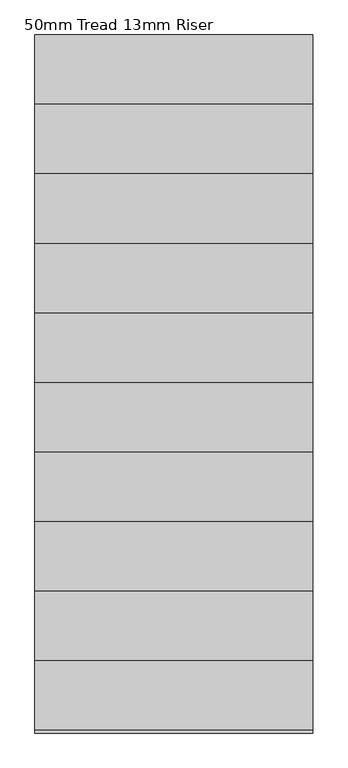
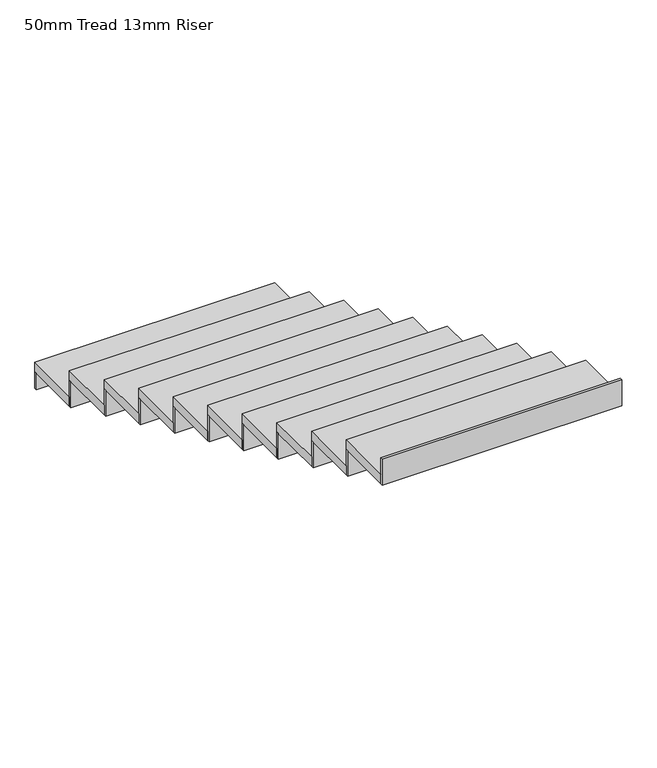
"""IFC4 building model written with IfcOpenShell, lengths in millimetres: stair flight geometry, 50mm Tread 13mm Riser."""

from ifc_helpers import new_model, si_unit, frame, origin, origin_with_axes, place, context, project, spatial, polyline, outline, extrude, source, transform, mapped, element, save


def stair_flight_50mm_tread_13mm_riser_f0aa37fc(model_context):
    return source(origin(), model_context, "Body", "SweptSolid", [
        extrude(outline(polyline([(21558.5156953, 793.6136739), (21558.5156953, 806.1136739), (22758.5156953, 806.1136739), (22758.5156953, 793.6136739), (21558.5156953, 793.6136739)])), origin_with_axes(), (0.0, 0.0, 1.0), 86.3636364),
        extrude(outline(polyline([(22758.5156953, 506.1136739), (21558.5156953, 506.1136739), (21558.5156953, 806.1136739), (22758.5156953, 806.1136739), (22758.5156953, 506.1136739)])), frame((0.0, 0.0, 86.3636364), z_axis=(0.0, 0.0, 1.0), x_axis=(1.0, 0.0, 0.0)), (0.0, 0.0, 1.0), 50.0),
        extrude(outline(polyline([(21558.5156953, 493.6136739), (21558.5156953, 506.1136739), (22758.5156953, 506.1136739), (22758.5156953, 493.6136739), (21558.5156953, 493.6136739)])), frame((0.0, 0.0, 86.3636364), z_axis=(0.0, 0.0, 1.0), x_axis=(1.0, 0.0, 0.0)), (0.0, 0.0, 1.0), 136.3636364),
        extrude(outline(polyline([(22758.5156953, 206.1136739), (21558.5156953, 206.1136739), (21558.5156953, 506.1136739), (22758.5156953, 506.1136739), (22758.5156953, 206.1136739)])), frame((0.0, 0.0, 222.7272727), z_axis=(0.0, 0.0, 1.0), x_axis=(1.0, 0.0, 0.0)), (0.0, 0.0, 1.0), 50.0),
        extrude(outline(polyline([(21558.5156953, 193.6136739), (21558.5156953, 206.1136739), (22758.5156953, 206.1136739), (22758.5156953, 193.6136739), (21558.5156953, 193.6136739)])), frame((0.0, 0.0, 222.7272727), z_axis=(0.0, 0.0, 1.0), x_axis=(1.0, 0.0, 0.0)), (0.0, 0.0, 1.0), 136.3636364),
        extrude(outline(polyline([(22758.5156953, -93.8863261), (21558.5156953, -93.8863261), (21558.5156953, 206.1136739), (22758.5156953, 206.1136739), (22758.5156953, -93.8863261)])), frame((0.0, 0.0, 359.0909091), z_axis=(0.0, 0.0, 1.0), x_axis=(1.0, 0.0, 0.0)), (0.0, 0.0, 1.0), 50.0),
        extrude(outline(polyline([(21558.5156953, -106.3863261), (21558.5156953, -93.8863261), (22758.5156953, -93.8863261), (22758.5156953, -106.3863261), (21558.5156953, -106.3863261)])), frame((0.0, 0.0, 359.0909091), z_axis=(0.0, 0.0, 1.0), x_axis=(1.0, 0.0, 0.0)), (0.0, 0.0, 1.0), 136.3636364),
        extrude(outline(polyline([(22758.5156953, -393.8863261), (21558.5156953, -393.8863261), (21558.5156953, -93.8863261), (22758.5156953, -93.8863261), (22758.5156953, -393.8863261)])), frame((0.0, 0.0, 495.4545455), z_axis=(0.0, 0.0, 1.0), x_axis=(1.0, 0.0, 0.0)), (0.0, 0.0, 1.0), 50.0),
        extrude(outline(polyline([(21558.5156953, -406.3863261), (21558.5156953, -393.8863261), (22758.5156953, -393.8863261), (22758.5156953, -406.3863261), (21558.5156953, -406.3863261)])), frame((0.0, 0.0, 495.4545455), z_axis=(0.0, 0.0, 1.0), x_axis=(1.0, 0.0, 0.0)), (0.0, 0.0, 1.0), 136.3636364),
        extrude(outline(polyline([(22758.5156953, -693.8863261), (21558.5156953, -693.8863261), (21558.5156953, -393.8863261), (22758.5156953, -393.8863261), (22758.5156953, -693.8863261)])), frame((0.0, 0.0, 631.8181818), z_axis=(0.0, 0.0, 1.0), x_axis=(1.0, 0.0, 0.0)), (0.0, 0.0, 1.0), 50.0),
        extrude(outline(polyline([(21558.5156953, -706.3863261), (21558.5156953, -693.8863261), (22758.5156953, -693.8863261), (22758.5156953, -706.3863261), (21558.5156953, -706.3863261)])), frame((0.0, 0.0, 631.8181818), z_axis=(0.0, 0.0, 1.0), x_axis=(1.0, 0.0, 0.0)), (0.0, 0.0, 1.0), 136.3636364),
        extrude(outline(polyline([(22758.5156953, -993.8863261), (21558.5156953, -993.8863261), (21558.5156953, -693.8863261), (22758.5156953, -693.8863261), (22758.5156953, -993.8863261)])), frame((0.0, 0.0, 768.1818182), z_axis=(0.0, 0.0, 1.0), x_axis=(1.0, 0.0, 0.0)), (0.0, 0.0, 1.0), 50.0),
        extrude(outline(polyline([(21558.5156953, -1006.3863261), (21558.5156953, -993.8863261), (22758.5156953, -993.8863261), (22758.5156953, -1006.3863261), (21558.5156953, -1006.3863261)])), frame((0.0, 0.0, 768.1818182), z_axis=(0.0, 0.0, 1.0), x_axis=(1.0, 0.0, 0.0)), (0.0, 0.0, 1.0), 136.3636364),
        extrude(outline(polyline([(22758.5156953, -1293.8863261), (21558.5156953, -1293.8863261), (21558.5156953, -993.8863261), (22758.5156953, -993.8863261), (22758.5156953, -1293.8863261)])), frame((0.0, 0.0, 904.5454545), z_axis=(0.0, 0.0, 1.0), x_axis=(1.0, 0.0, 0.0)), (0.0, 0.0, 1.0), 50.0),
        extrude(outline(polyline([(21558.5156953, -1306.3863261), (21558.5156953, -1293.8863261), (22758.5156953, -1293.8863261), (22758.5156953, -1306.3863261), (21558.5156953, -1306.3863261)])), frame((0.0, 0.0, 904.5454545), z_axis=(0.0, 0.0, 1.0), x_axis=(1.0, 0.0, 0.0)), (0.0, 0.0, 1.0), 136.3636364),
        extrude(outline(polyline([(22758.5156953, -1593.8863261), (21558.5156953, -1593.8863261), (21558.5156953, -1293.8863261), (22758.5156953, -1293.8863261), (22758.5156953, -1593.8863261)])), frame((0.0, 0.0, 1040.9090909), z_axis=(0.0, 0.0, 1.0), x_axis=(1.0, 0.0, 0.0)), (0.0, 0.0, 1.0), 50.0),
        extrude(outline(polyline([(21558.5156953, -1606.3863261), (21558.5156953, -1593.8863261), (22758.5156953, -1593.8863261), (22758.5156953, -1606.3863261), (21558.5156953, -1606.3863261)])), frame((0.0, 0.0, 1040.9090909), z_axis=(0.0, 0.0, 1.0), x_axis=(1.0, 0.0, 0.0)), (0.0, 0.0, 1.0), 136.3636364),
        extrude(outline(polyline([(22758.5156953, -1893.8863261), (21558.5156953, -1893.8863261), (21558.5156953, -1593.8863261), (22758.5156953, -1593.8863261), (22758.5156953, -1893.8863261)])), frame((0.0, 0.0, 1177.2727273), z_axis=(0.0, 0.0, 1.0), x_axis=(1.0, 0.0, 0.0)), (0.0, 0.0, 1.0), 50.0),
        extrude(outline(polyline([(21558.5156953, -1906.3863261), (21558.5156953, -1893.8863261), (22758.5156953, -1893.8863261), (22758.5156953, -1906.3863261), (21558.5156953, -1906.3863261)])), frame((0.0, 0.0, 1177.2727273), z_axis=(0.0, 0.0, 1.0), x_axis=(1.0, 0.0, 0.0)), (0.0, 0.0, 1.0), 136.3636364),
        extrude(outline(polyline([(21558.5156953, -2206.3863261), (21558.5156953, -2193.8863261), (22758.5156953, -2193.8863261), (22758.5156953, -2206.3863261), (21558.5156953, -2206.3863261)])), frame((0.0, 0.0, 1313.6363636), z_axis=(0.0, 0.0, 1.0), x_axis=(1.0, 0.0, 0.0)), (0.0, 0.0, 1.0), 136.3636364),
        extrude(outline(polyline([(22758.5156953, -2193.8863261), (21558.5156953, -2193.8863261), (21558.5156953, -1893.8863261), (22758.5156953, -1893.8863261), (22758.5156953, -2193.8863261)])), frame((0.0, 0.0, 1313.6363636), z_axis=(0.0, 0.0, 1.0), x_axis=(1.0, 0.0, 0.0)), (0.0, 0.0, 1.0), 50.0),
    ])


if __name__ == "__main__":
    model = new_model("IFC4")
    model_context = context("Model", 3, world=origin())
    ifc_project = project(units=[si_unit("LENGTHUNIT", "METRE", prefix="MILLI")], contexts=[model_context])
    site = spatial("IfcSite", under=ifc_project)
    building = spatial("IfcBuilding", under=site)
    placement = place(None, origin())
    stair_flight_50mm_tread_13mm_riser_shape = stair_flight_50mm_tread_13mm_riser_f0aa37fc(model_context)
    element("IfcStairFlight", 1, ObjectType="50mm Tread 13mm Riser", at=placement, inside=building, context=model_context, shape_type="MappedRepresentation", body=[
        mapped(stair_flight_50mm_tread_13mm_riser_shape, transform((0.0, 0.0, 0.0), x_axis=(1.0, 0.0, 0.0), y_axis=(0.0, 1.0, 0.0), z_axis=(0.0, 0.0, 1.0))),
    ])
    save(model, "model.ifc")
